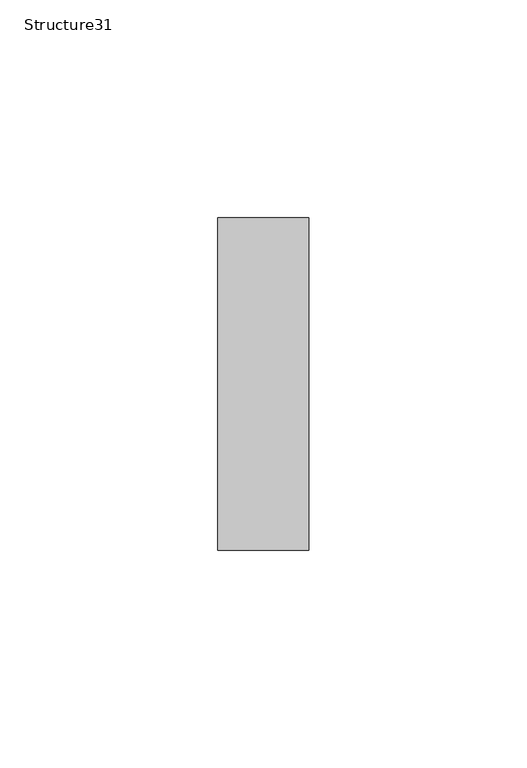
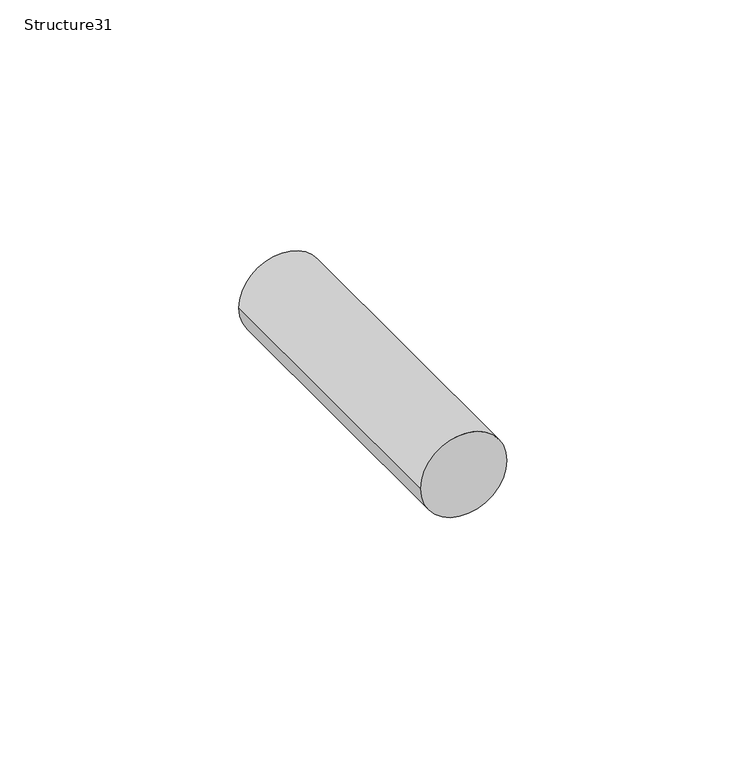
"""IFC4 building model written with IfcOpenShell, lengths in millimetres: proxy geometry, Structure31 : Structure668217129."""

from ifc_helpers import new_model, si_unit, point, frame, frame_2d, origin, place, context, project, spatial, circle_curve, trimmed, segment, composite_curve, outline, extrude, source, transform, mapped, element, save


def structure31_bf5528e4(model_context):
    return source(origin(), model_context, "Body", "SweptSolid", [
        extrude(outline(composite_curve([segment(trimmed(circle_curve(frame_2d((39371.6422813, 7343.0332877)), 10.4009751), [point((39371.6422813, 7332.6323126))], [point((39371.6422813, 7353.4342628))], False, "CARTESIAN"), True, "CONTINUOUS"), segment(trimmed(circle_curve(frame_2d((39371.6422813, 7343.0332877)), 10.4009751), [point((39371.6422813, 7353.4342628))], [point((39371.6422813, 7332.6323126))], False, "CARTESIAN"), True, "CONTINUOUS")], self_intersect=False)), frame((0.0, 933.5121669, 0.0), z_axis=(0.0, 1.0, 0.0), x_axis=(0.0, 0.0, 1.0)), (0.0, 0.0, 1.0), 76.2),
    ])


if __name__ == "__main__":
    model = new_model("IFC4")
    model_context = context("Model", 3, world=origin())
    ifc_project = project(units=[si_unit("LENGTHUNIT", "METRE", prefix="MILLI")], contexts=[model_context])
    site = spatial("IfcSite", under=ifc_project)
    building = spatial("IfcBuilding", under=site)
    placement = place(None, origin())
    structure31_shape = structure31_bf5528e4(model_context)
    element("IfcBuildingElementProxy", 1, Name="Structure31 : Structure668217129", ObjectType="Structure31 : Structure668217129", at=placement, inside=building, context=model_context, shape_type="MappedRepresentation", body=[
        mapped(structure31_shape, transform((0.0, 0.0, 0.0), x_axis=(1.0, 0.0, 0.0), y_axis=(0.0, 1.0, 0.0), z_axis=(0.0, 0.0, 1.0))),
    ])
    save(model, "model.ifc")

# Revit data of these elements
# Type "Structure31 : Structure668217129"
#   NameOverride = "Structure668217129"
# Element 1 (IfcBuildingElementProxy, "Structure31 : Structure668217129")
#   Materials on its faces: "1.5\" DIA. STAINLESS STEEL RAILING"
# Materials
#   "1.5\" DIA. STAINLESS STEEL RAILING": class "Unassigned", colour RGB 128 128 128, transparency 0, Cost = 0
